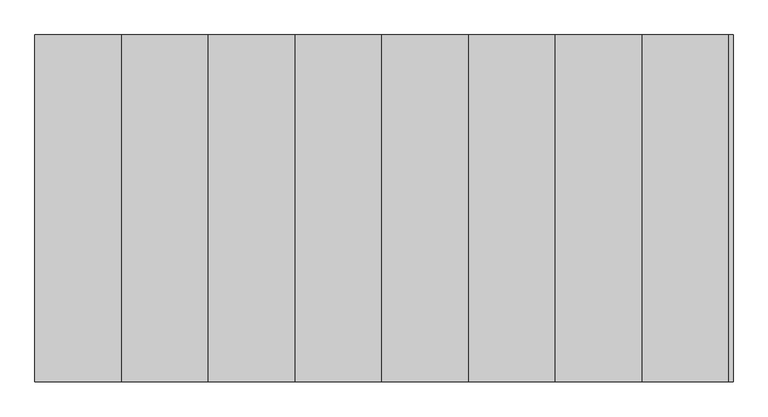
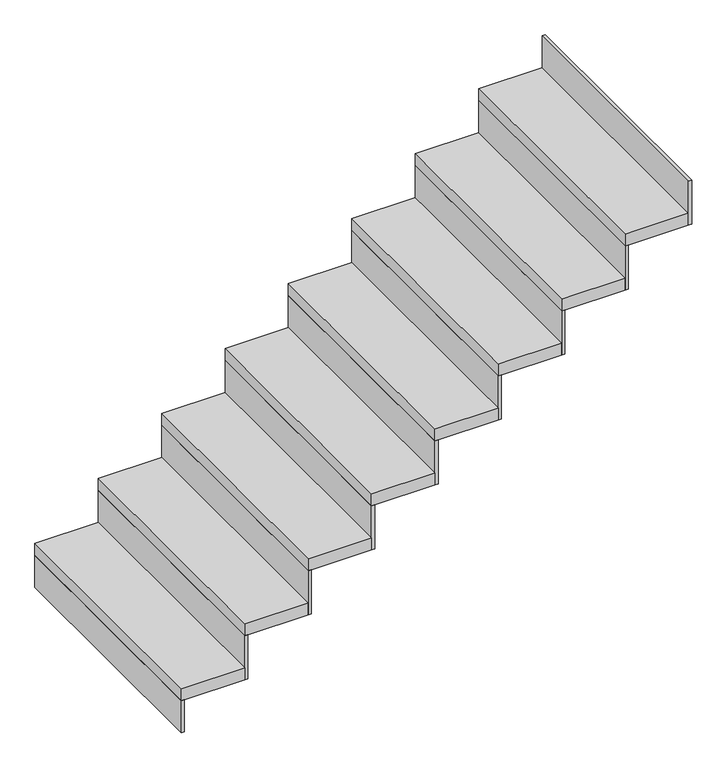
"""IFC4 building model written with IfcOpenShell, lengths in millimetres: stair flight geometry."""

import ifcopenshell
import ifcopenshell.guid

model = None  # the IFC model being written
_history = None  # IfcOwnerHistory: only IFC2X3 demands one
_inside = {}  # id of a spatial element -> (the spatial element, [elements in it])
_under = {}  # id of a project, library or spatial element -> (it, [spatial elements below it])
_declared = {}  # id of a project -> (the project, [libraries it declares])
_typed = {}  # id of a type object -> (the type object, [elements of that type])
_made_of = {}  # id of a material, layer set ... -> (it, [elements and type objects made of it])


def new_model(schema):
    """Start an empty IFC model of exactly this schema.

    Asked for "IFC4X3", IfcOpenShell would pick the latest addendum, in which some entities
    have other attributes; the version numbers below select the first issue.
    IFC2X3 requires an IfcOwnerHistory on every rooted entity: one is made here for all.
    """
    global model, _history
    if schema == "IFC4X3":
        model = ifcopenshell.file(schema_version=(4, 3, 0, 0))
    else:
        model = ifcopenshell.file(schema=schema)
    _inside.clear()
    _under.clear()
    _declared.clear()
    _typed.clear()
    _made_of.clear()
    _history = None
    if model.schema == "IFC2X3":
        org = make("IfcOrganization", Name="unknown")
        user = make(
            "IfcPersonAndOrganization",
            ThePerson=make("IfcPerson", FamilyName="unknown"),
            TheOrganization=org,
        )
        app = make(
            "IfcApplication",
            ApplicationDeveloper=org,
            Version="unknown",
            ApplicationFullName="unknown",
            ApplicationIdentifier="unknown",
        )
        _history = make(
            "IfcOwnerHistory",
            OwningUser=user,
            OwningApplication=app,
            ChangeAction="ADDED",
            CreationDate=0,
        )
    return model


def make(cls, **values):
    """One entity of the class cls with the attributes given. An attribute that is None is left unset."""
    return model.create_entity(
        cls, **{name: value for name, value in values.items() if value is not None}
    )


def rooted(cls, **values):
    """An entity with a GlobalId (a new one), such as an element, a storey or a relation."""
    return make(cls, GlobalId=ifcopenshell.guid.new(), OwnerHistory=_history, **values)


def si_unit(unit_type, name, prefix=None):
    """IfcSIUnit, for example si_unit("LENGTHUNIT", "METRE", prefix="MILLI")."""
    return make("IfcSIUnit", UnitType=unit_type, Prefix=prefix, Name=name)


def assignment(units):
    """IfcUnitAssignment: the units of a project."""
    return None if units is None else make("IfcUnitAssignment", Units=units)


def point(xyz):
    """IfcCartesianPoint."""
    return None if xyz is None else make("IfcCartesianPoint", Coordinates=xyz)


def direction(xyz):
    """IfcDirection."""
    return None if xyz is None else make("IfcDirection", DirectionRatios=xyz)


def frame(location, z_axis=None, x_axis=None):
    """IfcAxis2Placement3D, a coordinate frame: its origin and axes. An axis left out is left unset."""
    return make(
        "IfcAxis2Placement3D",
        Location=point(location),
        Axis=direction(z_axis),
        RefDirection=direction(x_axis),
    )


def origin():
    """The frame at (0, 0, 0) with its axes left unset."""
    return frame((0.0, 0.0, 0.0))


def origin_with_axes():
    """The frame at (0, 0, 0) with the z axis (0, 0, 1) and the x axis (1, 0, 0) written out."""
    return frame((0.0, 0.0, 0.0), z_axis=(0.0, 0.0, 1.0), x_axis=(1.0, 0.0, 0.0))


def place(relative_to, where):
    """IfcLocalPlacement: puts the frame where relative to a parent placement (None: the world)."""
    return make(
        "IfcLocalPlacement", PlacementRelTo=relative_to, RelativePlacement=where
    )


def context(
    kind, dimensions, precision=None, world=None, true_north=None, identifier=None
):
    """IfcGeometricRepresentationContext, for example the 3D "Model" context."""
    return make(
        "IfcGeometricRepresentationContext",
        ContextIdentifier=identifier,
        ContextType=kind,
        CoordinateSpaceDimension=dimensions,
        Precision=precision,
        WorldCoordinateSystem=world,
        TrueNorth=true_north,
    )


def project(units=None, contexts=None):
    """IfcProject with its units and contexts."""
    return rooted(
        "IfcProject",
        Name="project",
        RepresentationContexts=contexts,
        UnitsInContext=assignment(units),
    )


def spatial(cls, under=None, at=None, **own):
    """A site, building, storey or space (cls), placed at a placement, below another one or the project."""
    s = rooted(cls, ObjectPlacement=at, **own)
    if under is not None:
        _under.setdefault(under.id(), (under, []))[1].append(s)
    return s


def polyline(points):
    """IfcPolyline through the points."""
    return make("IfcPolyline", Points=[point(p) for p in points])


def outline(outer, holes=None, kind="AREA"):
    """IfcArbitraryClosedProfileDef: a profile drawn as a closed curve; with holes, ...WithVoids."""
    if holes is None:
        return make("IfcArbitraryClosedProfileDef", ProfileType=kind, OuterCurve=outer)
    return make(
        "IfcArbitraryProfileDefWithVoids",
        ProfileType=kind,
        OuterCurve=outer,
        InnerCurves=holes,
    )


def extrude(swept, where, along, depth):
    """IfcExtrudedAreaSolid: the profile swept, set in the frame where, extruded along a direction by depth."""
    return make(
        "IfcExtrudedAreaSolid",
        SweptArea=swept,
        Position=where,
        ExtrudedDirection=direction(along),
        Depth=depth,
    )


def shape(context_of_items, identifier, shape_type, items):
    """IfcShapeRepresentation: the items that make up one representation, for example the "Body"."""
    return make(
        "IfcShapeRepresentation",
        ContextOfItems=context_of_items,
        RepresentationIdentifier=identifier,
        RepresentationType=shape_type,
        Items=items,
    )


def source(mapping_origin, context_of_items, identifier, shape_type, items):
    """IfcRepresentationMap: a shape defined once, which mapped items show again and again."""
    return make(
        "IfcRepresentationMap",
        MappingOrigin=mapping_origin,
        MappedRepresentation=shape(context_of_items, identifier, shape_type, items),
    )


def transform(
    local_origin,
    x_axis=None,
    y_axis=None,
    z_axis=None,
    scale=None,
    scale2=None,
    scale3=None,
    uniform=True,
):
    """IfcCartesianTransformationOperator3D, or its non-uniform kind. x_axis, y_axis, z_axis: its Axis1, 2, 3."""
    if uniform:
        return make(
            "IfcCartesianTransformationOperator3D",
            Axis1=direction(x_axis),
            Axis2=direction(y_axis),
            LocalOrigin=point(local_origin),
            Scale=scale,
            Axis3=direction(z_axis),
        )
    return make(
        "IfcCartesianTransformationOperator3DnonUniform",
        Axis1=direction(x_axis),
        Axis2=direction(y_axis),
        LocalOrigin=point(local_origin),
        Scale=scale,
        Axis3=direction(z_axis),
        Scale2=scale2,
        Scale3=scale3,
    )


def mapped(mapping_source, mapping_target):
    """IfcMappedItem: shows the shape of a source again, moved by a transform."""
    return make(
        "IfcMappedItem", MappingSource=mapping_source, MappingTarget=mapping_target
    )


def made_of(thing, what):
    """Note that an element or type object is made of a material, layer set ...; save() writes the relation."""
    if what is not None:
        _made_of.setdefault(what.id(), (what, []))[1].append(thing)
    return thing


def element(
    cls,
    number,
    at=None,
    inside=None,
    cuts=None,
    type_object=None,
    material=None,
    context=None,
    identifier="Body",
    shape_type=None,
    held_by="IfcProductDefinitionShape",
    body=None,
    shapes=None,
    **own,
):
    """One element of the class cls, such as IfcWall. Its Tag is "e" and its number.

    at: its placement. inside: the storey or other place that contains it. cuts: it is an
    opening in that element (IfcRelVoidsElement). A single representation is given by context,
    identifier, shape_type and body (its items); several are given by shapes. held_by: the class
    of the entity that holds the representations. save() writes the other relations.
    """
    e = rooted(cls, Tag="e%d" % number, ObjectPlacement=at, **own)
    if body is not None:
        shapes = [shape(context, identifier, shape_type, body)]
    if shapes is not None:
        e.Representation = make(held_by, Representations=shapes)
    if inside is not None:
        _inside.setdefault(inside.id(), (inside, []))[1].append(e)
    if cuts is not None:
        rooted(
            "IfcRelVoidsElement", RelatingBuildingElement=cuts, RelatedOpeningElement=e
        )
    if type_object is not None:
        _typed.setdefault(type_object.id(), (type_object, []))[1].append(e)
    return made_of(e, material)


def aggregate(whole, parts):
    """IfcRelAggregates: a whole, such as a stair, and the parts it consists of."""
    return rooted("IfcRelAggregates", RelatingObject=whole, RelatedObjects=parts)


def save(model, path):
    """Write the relations noted so far, then the file.

    IfcRelAggregates (storeys below a building ...), IfcRelContainedInSpatialStructure (elements
    in a storey), IfcRelDefinesByType, IfcRelAssociatesMaterial and IfcRelDeclares: one each for
    every whole, place, type object, material and project.
    """
    for whole, parts in _under.values():
        aggregate(whole, parts)
    for where, things in _inside.values():
        rooted(
            "IfcRelContainedInSpatialStructure",
            RelatedElements=things,
            RelatingStructure=where,
        )
    for kind, things in _typed.values():
        rooted("IfcRelDefinesByType", RelatedObjects=things, RelatingType=kind)
    for what, things in _made_of.values():
        rooted("IfcRelAssociatesMaterial", RelatedObjects=things, RelatingMaterial=what)
    for by, libraries in _declared.values():
        rooted("IfcRelDeclares", RelatingContext=by, RelatedDefinitions=libraries)
    model.write(path)


def stair_flight_23111021(model_context):
    return source(origin(), model_context, "Body", "SweptSolid", [
        extrude(outline(polyline([(3289.0556606, 2685.7983707), (3276.5556606, 2685.7983707), (3276.5556606, 3685.7983707), (3289.0556606, 3685.7983707), (3289.0556606, 2685.7983707)])), origin_with_axes(), (0.0, 0.0, 1.0), 133.3333333),
        extrude(outline(polyline([(3526.5556606, 3685.7983707), (3526.5556606, 2685.7983707), (3276.5556606, 2685.7983707), (3276.5556606, 3685.7983707), (3526.5556606, 3685.7983707)])), frame((0.0, 0.0, 133.3333333), z_axis=(0.0, 0.0, 1.0), x_axis=(1.0, 0.0, 0.0)), (0.0, 0.0, 1.0), 50.0),
        extrude(outline(polyline([(3539.0556606, 2685.7983707), (3526.5556606, 2685.7983707), (3526.5556606, 3685.7983707), (3539.0556606, 3685.7983707), (3539.0556606, 2685.7983707)])), frame((0.0, 0.0, 133.3333333), z_axis=(0.0, 0.0, 1.0), x_axis=(1.0, 0.0, 0.0)), (0.0, 0.0, 1.0), 183.3333333),
        extrude(outline(polyline([(3776.5556606, 3685.7983707), (3776.5556606, 2685.7983707), (3526.5556606, 2685.7983707), (3526.5556606, 3685.7983707), (3776.5556606, 3685.7983707)])), frame((0.0, 0.0, 316.6666667), z_axis=(0.0, 0.0, 1.0), x_axis=(1.0, 0.0, 0.0)), (0.0, 0.0, 1.0), 50.0),
        extrude(outline(polyline([(3789.0556606, 2685.7983707), (3776.5556606, 2685.7983707), (3776.5556606, 3685.7983707), (3789.0556606, 3685.7983707), (3789.0556606, 2685.7983707)])), frame((0.0, 0.0, 316.6666667), z_axis=(0.0, 0.0, 1.0), x_axis=(1.0, 0.0, 0.0)), (0.0, 0.0, 1.0), 183.3333333),
        extrude(outline(polyline([(4026.5556606, 3685.7983707), (4026.5556606, 2685.7983707), (3776.5556606, 2685.7983707), (3776.5556606, 3685.7983707), (4026.5556606, 3685.7983707)])), frame((0.0, 0.0, 500.0), z_axis=(0.0, 0.0, 1.0), x_axis=(1.0, 0.0, 0.0)), (0.0, 0.0, 1.0), 50.0),
        extrude(outline(polyline([(4039.0556606, 2685.7983707), (4026.5556606, 2685.7983707), (4026.5556606, 3685.7983707), (4039.0556606, 3685.7983707), (4039.0556606, 2685.7983707)])), frame((0.0, 0.0, 500.0), z_axis=(0.0, 0.0, 1.0), x_axis=(1.0, 0.0, 0.0)), (0.0, 0.0, 1.0), 183.3333333),
        extrude(outline(polyline([(4276.5556606, 3685.7983707), (4276.5556606, 2685.7983707), (4026.5556606, 2685.7983707), (4026.5556606, 3685.7983707), (4276.5556606, 3685.7983707)])), frame((0.0, 0.0, 683.3333333), z_axis=(0.0, 0.0, 1.0), x_axis=(1.0, 0.0, 0.0)), (0.0, 0.0, 1.0), 50.0),
        extrude(outline(polyline([(4289.0556606, 2685.7983707), (4276.5556606, 2685.7983707), (4276.5556606, 3685.7983707), (4289.0556606, 3685.7983707), (4289.0556606, 2685.7983707)])), frame((0.0, 0.0, 683.3333333), z_axis=(0.0, 0.0, 1.0), x_axis=(1.0, 0.0, 0.0)), (0.0, 0.0, 1.0), 183.3333333),
        extrude(outline(polyline([(4526.5556606, 3685.7983707), (4526.5556606, 2685.7983707), (4276.5556606, 2685.7983707), (4276.5556606, 3685.7983707), (4526.5556606, 3685.7983707)])), frame((0.0, 0.0, 866.6666667), z_axis=(0.0, 0.0, 1.0), x_axis=(1.0, 0.0, 0.0)), (0.0, 0.0, 1.0), 50.0),
        extrude(outline(polyline([(4539.0556606, 2685.7983707), (4526.5556606, 2685.7983707), (4526.5556606, 3685.7983707), (4539.0556606, 3685.7983707), (4539.0556606, 2685.7983707)])), frame((0.0, 0.0, 866.6666667), z_axis=(0.0, 0.0, 1.0), x_axis=(1.0, 0.0, 0.0)), (0.0, 0.0, 1.0), 183.3333333),
        extrude(outline(polyline([(4776.5556606, 3685.7983707), (4776.5556606, 2685.7983707), (4526.5556606, 2685.7983707), (4526.5556606, 3685.7983707), (4776.5556606, 3685.7983707)])), frame((0.0, 0.0, 1050.0), z_axis=(0.0, 0.0, 1.0), x_axis=(1.0, 0.0, 0.0)), (0.0, 0.0, 1.0), 50.0),
        extrude(outline(polyline([(4789.0556606, 2685.7983707), (4776.5556606, 2685.7983707), (4776.5556606, 3685.7983707), (4789.0556606, 3685.7983707), (4789.0556606, 2685.7983707)])), frame((0.0, 0.0, 1050.0), z_axis=(0.0, 0.0, 1.0), x_axis=(1.0, 0.0, 0.0)), (0.0, 0.0, 1.0), 183.3333333),
        extrude(outline(polyline([(5026.5556606, 3685.7983707), (5026.5556606, 2685.7983707), (4776.5556606, 2685.7983707), (4776.5556606, 3685.7983707), (5026.5556606, 3685.7983707)])), frame((0.0, 0.0, 1233.3333333), z_axis=(0.0, 0.0, 1.0), x_axis=(1.0, 0.0, 0.0)), (0.0, 0.0, 1.0), 50.0),
        extrude(outline(polyline([(5039.0556606, 2685.7983707), (5026.5556606, 2685.7983707), (5026.5556606, 3685.7983707), (5039.0556606, 3685.7983707), (5039.0556606, 2685.7983707)])), frame((0.0, 0.0, 1233.3333333), z_axis=(0.0, 0.0, 1.0), x_axis=(1.0, 0.0, 0.0)), (0.0, 0.0, 1.0), 183.3333333),
        extrude(outline(polyline([(5289.0556606, 2685.7983707), (5276.5556606, 2685.7983707), (5276.5556606, 3685.7983707), (5289.0556606, 3685.7983707), (5289.0556606, 2685.7983707)])), frame((0.0, 0.0, 1416.6666667), z_axis=(0.0, 0.0, 1.0), x_axis=(1.0, 0.0, 0.0)), (0.0, 0.0, 1.0), 183.3333333),
        extrude(outline(polyline([(5276.5556606, 3685.7983707), (5276.5556606, 2685.7983707), (5026.5556606, 2685.7983707), (5026.5556606, 3685.7983707), (5276.5556606, 3685.7983707)])), frame((0.0, 0.0, 1416.6666667), z_axis=(0.0, 0.0, 1.0), x_axis=(1.0, 0.0, 0.0)), (0.0, 0.0, 1.0), 50.0),
    ])


if __name__ == "__main__":
    model = new_model("IFC4")
    model_context = context("Model", 3, world=origin())
    ifc_project = project(units=[si_unit("LENGTHUNIT", "METRE", prefix="MILLI")], contexts=[model_context])
    site = spatial("IfcSite", under=ifc_project)
    building = spatial("IfcBuilding", under=site)
    placement = place(None, origin())
    stair_flight_shape = stair_flight_23111021(model_context)
    element("IfcStairFlight", 1, at=placement, inside=building, context=model_context, shape_type="MappedRepresentation", body=[
        mapped(stair_flight_shape, transform((0.0, 0.0, 0.0), x_axis=(1.0, 0.0, 0.0), y_axis=(0.0, 1.0, 0.0), z_axis=(0.0, 0.0, 1.0))),
    ])
    save(model, "model.ifc")
